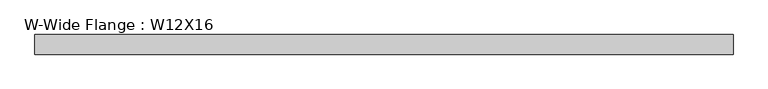
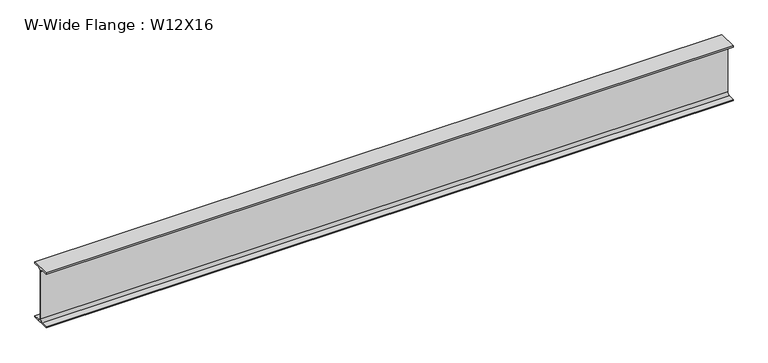
"""IFC4 building model written with IfcOpenShell, lengths in millimetres: beam geometry, W-Wide Flange : W12X16."""

from ifc_helpers import new_model, si_unit, point, frame, frame_2d, origin, place, context, project, spatial, polyline, circle_curve, trimmed, segment, composite_curve, outline, extrude, source, transform, mapped, element, save


def w_wide_flange_w12x16_d958fc51(model_context):
    return source(origin(), model_context, "Body", "SweptSolid", [
        extrude(outline(composite_curve([segment(polyline([(50.673, -145.669), (50.673, -152.4), (-50.673, -152.4), (-50.673, -145.669), (-16.7005, -145.669)]), True, "CONTINUOUS"), segment(trimmed(circle_curve(frame_2d((-16.7005, -131.7625)), 13.9065), [point((-16.7005, -145.669))], [point((-2.794, -131.7625))], True, "CARTESIAN"), True, "CONTINUOUS"), segment(polyline([(-2.794, -131.7625), (-2.794, 131.7625)]), True, "CONTINUOUS"), segment(trimmed(circle_curve(frame_2d((-16.7005, 131.7625)), 13.9065), [point((-2.794, 131.7625))], [point((-16.7005, 145.669))], True, "CARTESIAN"), True, "CONTINUOUS"), segment(polyline([(-16.7005, 145.669), (-50.673, 145.669), (-50.673, 152.4), (50.673, 152.4), (50.673, 145.669), (16.7005, 145.669)]), True, "CONTINUOUS"), segment(trimmed(circle_curve(frame_2d((16.7005, 131.7625)), 13.9065), [point((16.7005, 145.669))], [point((2.794, 131.7625))], True, "CARTESIAN"), True, "CONTINUOUS"), segment(polyline([(2.794, 131.7625), (2.794, -131.7625)]), True, "CONTINUOUS"), segment(trimmed(circle_curve(frame_2d((16.7005, -131.7625)), 13.9065), [point((2.794, -131.7625))], [point((16.7005, -145.669))], True, "CARTESIAN"), True, "CONTINUOUS"), segment(polyline([(16.7005, -145.669), (50.673, -145.669)]), True, "CONTINUOUS")], self_intersect=False)), frame((-1803.4, 0.0, 0.0), z_axis=(1.0, 0.0, 0.0), x_axis=(0.0, 1.0, 0.0)), (0.0, 0.0, 1.0), 3606.8),
    ])


if __name__ == "__main__":
    model = new_model("IFC4")
    model_context = context("Model", 3, world=origin())
    ifc_project = project(units=[si_unit("LENGTHUNIT", "METRE", prefix="MILLI")], contexts=[model_context])
    site = spatial("IfcSite", under=ifc_project)
    building = spatial("IfcBuilding", under=site)
    placement = place(None, origin())
    w_wide_flange_w12x16_shape = w_wide_flange_w12x16_d958fc51(model_context)
    element("IfcBeam", 1, ObjectType="W-Wide Flange : W12X16", at=placement, inside=building, context=model_context, shape_type="MappedRepresentation", body=[
        mapped(w_wide_flange_w12x16_shape, transform((0.0, 0.0, 0.0), x_axis=(1.0, 0.0, 0.0), y_axis=(0.0, 1.0, 0.0), z_axis=(0.0, 0.0, 1.0))),
    ])
    save(model, "model.ifc")

# Revit data of these elements
# Type "W-Wide Flange : W12X16"
#   Assembly Code = "B10"
#   W = 16
#   Length [instance default] = 5' - 0"
#   bf = 0' - 3.99"
#   d = 1' - 0"
#   k = 0' - 0 13/16"
#   k2 = 0' - 0.5475"
#   tf = 0' - 0.265"
#   tw = 0' - 0.22"
#   A = 0.0327083 SF
#   Structural Material [instance default] = Steel ASTM A992
# Element 1 (IfcBeam, "W-Wide Flange : W12X16")
#   Materials on its faces: "Steel ASTM A992"
# Materials
#   "Steel ASTM A992": class "Metal", colour RGB 199 199 199, transparency 0, Description = "Structural steel 50ksi", Cost = 0
